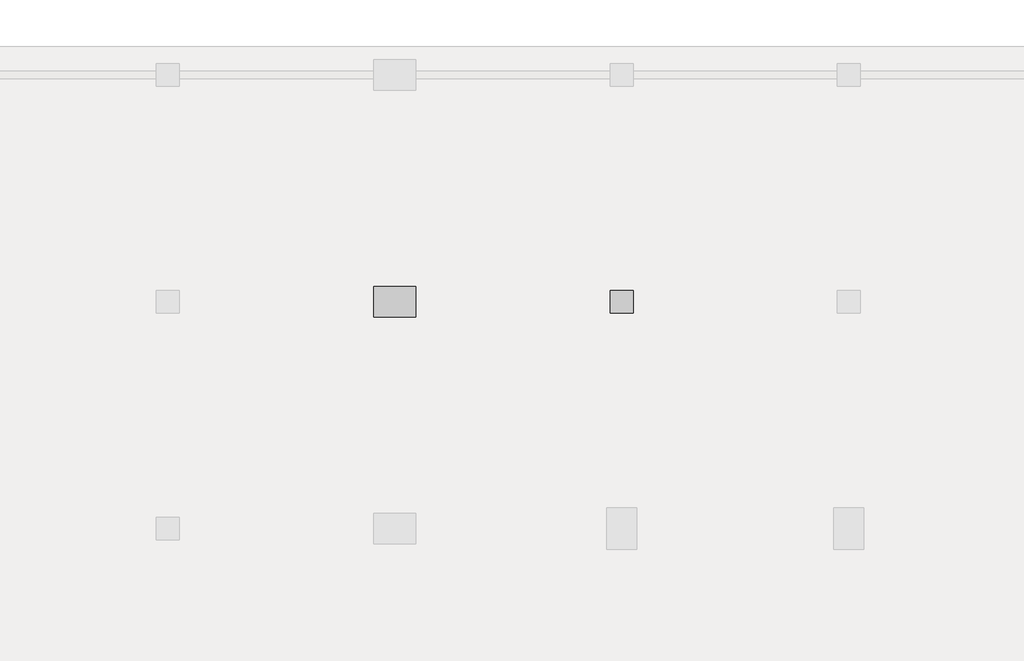
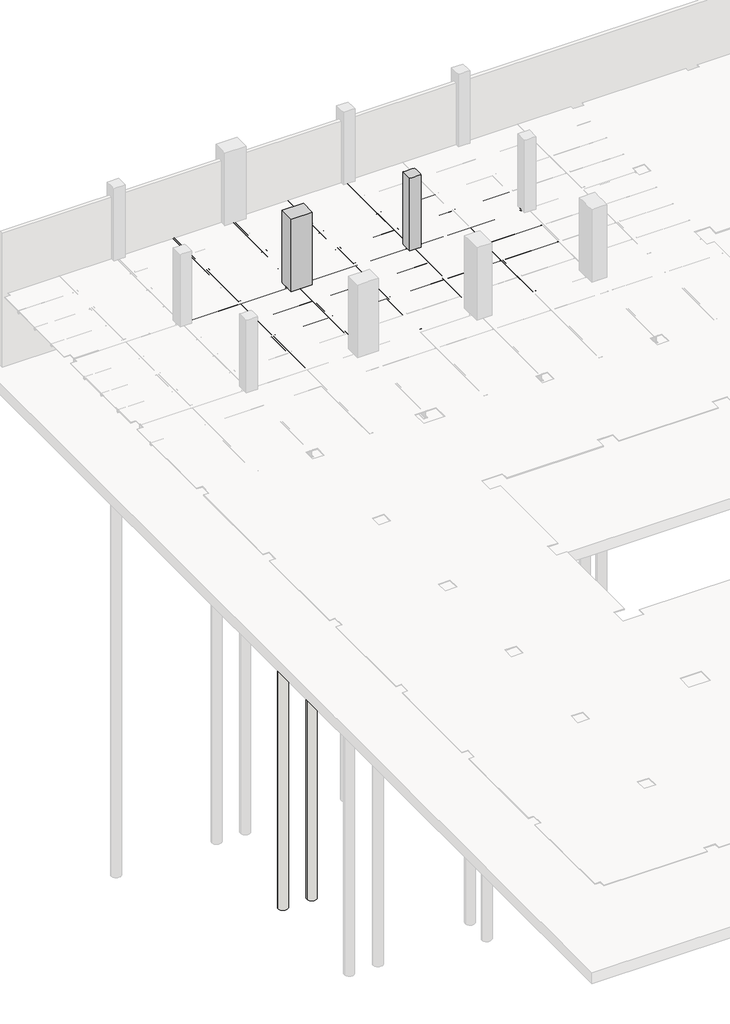
# Not in any storey, part 12 of 16: 31 beams, 2 columns, 2 slabs.
"""IFC4 building model written with IfcOpenShell, lengths in millimetres."""

from ifc_helpers import new_model, si_unit, point, frame, frame_2d, origin, place, context, project, spatial, polyline, circle_curve, trimmed, segment, composite_curve, outline, extrude, faceted_brep, element, save

model = new_model("IFC4")

# Units and contexts
model_context = context("Model", 3, world=origin())
ifc_project = project(units=[si_unit("LENGTHUNIT", "METRE", prefix="MILLI")], contexts=[model_context])

# Site, building
site = spatial("IfcSite", under=ifc_project)
building = spatial("IfcBuilding", under=site)

# Beams
placement = place(None, origin())
element("IfcBeam", 1, ObjectType="Steel Framing_H_KS : H_SB_AR_S02_H-400x200x8x13_BSG1", at=placement, inside=building, context=model_context, shape_type="SweptSolid", body=[
    extrude(outline(composite_curve([segment(polyline([(-11900.0, -4187.0381366), (-11900.0, -4200.0381366), (-12100.0, -4200.0381366), (-12100.0, -4187.0381366), (-12020.0, -4187.0381366)]), True, "CONTINUOUS"), segment(trimmed(circle_curve(frame_2d((-12020.0, -4171.0381366)), 16.0), [point((-12020.0, -4187.0381366))], [point((-12004.0, -4171.0381366))], True, "CARTESIAN"), True, "CONTINUOUS"), segment(polyline([(-12004.0, -4171.0381366), (-12004.0, -3829.0381366)]), True, "CONTINUOUS"), segment(trimmed(circle_curve(frame_2d((-12020.0, -3829.0381366)), 16.0), [point((-12004.0, -3829.0381366))], [point((-12020.0, -3813.0381366))], True, "CARTESIAN"), True, "CONTINUOUS"), segment(polyline([(-12020.0, -3813.0381366), (-12100.0, -3813.0381366), (-12100.0, -3800.0381366), (-11900.0, -3800.0381366), (-11900.0, -3813.0381366), (-11980.0, -3813.0381366)]), True, "CONTINUOUS"), segment(trimmed(circle_curve(frame_2d((-11980.0, -3829.0381366)), 16.0), [point((-11980.0, -3813.0381366))], [point((-11996.0, -3829.0381366))], True, "CARTESIAN"), True, "CONTINUOUS"), segment(polyline([(-11996.0, -3829.0381366), (-11996.0, -4171.0381366)]), True, "CONTINUOUS"), segment(trimmed(circle_curve(frame_2d((-11980.0, -4171.0381366)), 16.0), [point((-11996.0, -4171.0381366))], [point((-11980.0, -4187.0381366))], True, "CARTESIAN"), True, "CONTINUOUS"), segment(polyline([(-11980.0, -4187.0381366), (-11900.0, -4187.0381366)]), True, "CONTINUOUS")], self_intersect=False)), frame((30312.7, 0.0, 0.0), z_axis=(1.0, 0.0, 0.0), x_axis=(0.0, 1.0, 0.0)), (0.0, 0.0, 1.0), 5124.6),
])
element("IfcBeam", 2, ObjectType="Steel Framing_H_KS : H_SB_AR_S02_H-400x200x8x13_BSG2", at=placement, inside=building, context=model_context, shape_type="SweptSolid", body=[
    extrude(outline(composite_curve([segment(polyline([(-4187.0381366, 35900.0), (-4200.0381366, 35900.0), (-4200.0381366, 36100.0), (-4187.0381366, 36100.0), (-4187.0381366, 36020.0)]), True, "CONTINUOUS"), segment(trimmed(circle_curve(frame_2d((-4171.0381366, 36020.0)), 16.0), [point((-4187.0381366, 36020.0))], [point((-4171.0381366, 36004.0))], True, "CARTESIAN"), True, "CONTINUOUS"), segment(polyline([(-4171.0381366, 36004.0), (-3829.0381366, 36004.0)]), True, "CONTINUOUS"), segment(trimmed(circle_curve(frame_2d((-3829.0381366, 36020.0)), 16.0), [point((-3829.0381366, 36004.0))], [point((-3813.0381366, 36020.0))], True, "CARTESIAN"), True, "CONTINUOUS"), segment(polyline([(-3813.0381366, 36020.0), (-3813.0381366, 36100.0), (-3800.0381366, 36100.0), (-3800.0381366, 35900.0), (-3813.0381366, 35900.0), (-3813.0381366, 35980.0)]), True, "CONTINUOUS"), segment(trimmed(circle_curve(frame_2d((-3829.0381366, 35980.0)), 16.0), [point((-3813.0381366, 35980.0))], [point((-3829.0381366, 35996.0))], True, "CARTESIAN"), True, "CONTINUOUS"), segment(polyline([(-3829.0381366, 35996.0), (-4171.0381366, 35996.0)]), True, "CONTINUOUS"), segment(trimmed(circle_curve(frame_2d((-4171.0381366, 35980.0)), 16.0), [point((-4171.0381366, 35996.0))], [point((-4187.0381366, 35980.0))], True, "CARTESIAN"), True, "CONTINUOUS"), segment(polyline([(-4187.0381366, 35980.0), (-4187.0381366, 35900.0)]), True, "CONTINUOUS")], self_intersect=False)), frame((0.0, -11587.3, 0.0), z_axis=(0.0, 1.0, 0.0), x_axis=(0.0, 0.0, 1.0)), (0.0, 0.0, 1.0), 5174.6),
])
element("IfcBeam", 3, ObjectType="Steel Framing_H_KS : H_SB_AR_S02_H-400x200x8x13_BSB1", at=placement, inside=building, context=model_context, shape_type="SweptSolid", body=[
    extrude(outline(composite_curve([segment(polyline([(-4187.0381366, 32900.0), (-4200.0381366, 32900.0), (-4200.0381366, 33100.0), (-4187.0381366, 33100.0), (-4187.0381366, 33020.0)]), True, "CONTINUOUS"), segment(trimmed(circle_curve(frame_2d((-4171.0381366, 33020.0)), 16.0), [point((-4187.0381366, 33020.0))], [point((-4171.0381366, 33004.0))], True, "CARTESIAN"), True, "CONTINUOUS"), segment(polyline([(-4171.0381366, 33004.0), (-3829.0381366, 33004.0)]), True, "CONTINUOUS"), segment(trimmed(circle_curve(frame_2d((-3829.0381366, 33020.0)), 16.0), [point((-3829.0381366, 33004.0))], [point((-3813.0381366, 33020.0))], True, "CARTESIAN"), True, "CONTINUOUS"), segment(polyline([(-3813.0381366, 33020.0), (-3813.0381366, 33100.0), (-3800.0381366, 33100.0), (-3800.0381366, 32900.0), (-3813.0381366, 32900.0), (-3813.0381366, 32980.0)]), True, "CONTINUOUS"), segment(trimmed(circle_curve(frame_2d((-3829.0381366, 32980.0)), 16.0), [point((-3813.0381366, 32980.0))], [point((-3829.0381366, 32996.0))], True, "CARTESIAN"), True, "CONTINUOUS"), segment(polyline([(-3829.0381366, 32996.0), (-4171.0381366, 32996.0)]), True, "CONTINUOUS"), segment(trimmed(circle_curve(frame_2d((-4171.0381366, 32980.0)), 16.0), [point((-4171.0381366, 32996.0))], [point((-4187.0381366, 32980.0))], True, "CARTESIAN"), True, "CONTINUOUS"), segment(polyline([(-4187.0381366, 32980.0), (-4187.0381366, 32900.0)]), True, "CONTINUOUS")], self_intersect=False)), frame((0.0, -11887.3, 0.0), z_axis=(0.0, 1.0, 0.0), x_axis=(0.0, 0.0, 1.0)), (0.0, 0.0, 1.0), 5887.3),
])
element("IfcBeam", 4, ObjectType="Steel Framing_C_KS : H_SB_AR_S02_C-150x75x6.5x10_J1", at=placement, inside=building, context=model_context, shape_type="SweptSolid", body=[
    extrude(outline(composite_curve([segment(polyline([(-8977.2, -3800.0381366), (-8977.2, -3950.0381366), (-9052.2, -3950.0381366)]), True, "CONTINUOUS"), segment(trimmed(circle_curve(frame_2d((-9042.2, -3950.0381366)), 10.0), [point((-9052.2, -3950.0381366))], [point((-9042.2, -3940.0381366))], False, "CARTESIAN"), True, "CONTINUOUS"), segment(polyline([(-9042.2, -3940.0381366), (-8983.7, -3930.7726469), (-8983.7, -3819.3036264), (-9042.2, -3810.0381366)]), True, "CONTINUOUS"), segment(trimmed(circle_curve(frame_2d((-9042.2, -3800.0381366)), 10.0), [point((-9042.2, -3810.0381366))], [point((-9052.2, -3800.0381366))], False, "CARTESIAN"), True, "CONTINUOUS"), segment(polyline([(-9052.2, -3800.0381366), (-8977.2, -3800.0381366)]), True, "CONTINUOUS")], self_intersect=False)), frame((33112.7, 0.0, 0.0), z_axis=(1.0, 0.0, 0.0), x_axis=(0.0, 1.0, 0.0)), (0.0, 0.0, 1.0), 2774.6),
])
element("IfcBeam", 5, ObjectType="Steel Framing_C_KS : H_SB_AR_S02_C-150x75x6.5x10_J1", at=placement, inside=building, context=model_context, shape_type="SweptSolid", body=[
    extrude(outline(composite_curve([segment(polyline([(-10477.2, -3800.0381366), (-10477.2, -3950.0381366), (-10552.2, -3950.0381366)]), True, "CONTINUOUS"), segment(trimmed(circle_curve(frame_2d((-10542.2, -3950.0381366)), 10.0), [point((-10552.2, -3950.0381366))], [point((-10542.2, -3940.0381366))], False, "CARTESIAN"), True, "CONTINUOUS"), segment(polyline([(-10542.2, -3940.0381366), (-10483.7, -3930.7726469), (-10483.7, -3819.3036264), (-10542.2, -3810.0381366)]), True, "CONTINUOUS"), segment(trimmed(circle_curve(frame_2d((-10542.2, -3800.0381366)), 10.0), [point((-10542.2, -3810.0381366))], [point((-10552.2, -3800.0381366))], False, "CARTESIAN"), True, "CONTINUOUS"), segment(polyline([(-10552.2, -3800.0381366), (-10477.2, -3800.0381366)]), True, "CONTINUOUS")], self_intersect=False)), frame((33112.7, 0.0, 0.0), z_axis=(1.0, 0.0, 0.0), x_axis=(0.0, 1.0, 0.0)), (0.0, 0.0, 1.0), 2774.6),
])
element("IfcBeam", 6, ObjectType="Steel Framing_H_KS : H_SB_AR_S02_H-400x200x8x13_BSG1", at=placement, inside=building, context=model_context, shape_type="SweptSolid", body=[
    extrude(outline(composite_curve([segment(polyline([(-11900.0, -4187.0381366), (-11900.0, -4200.0381366), (-12100.0, -4200.0381366), (-12100.0, -4187.0381366), (-12020.0, -4187.0381366)]), True, "CONTINUOUS"), segment(trimmed(circle_curve(frame_2d((-12020.0, -4171.0381366)), 16.0), [point((-12020.0, -4187.0381366))], [point((-12004.0, -4171.0381366))], True, "CARTESIAN"), True, "CONTINUOUS"), segment(polyline([(-12004.0, -4171.0381366), (-12004.0, -3829.0381366)]), True, "CONTINUOUS"), segment(trimmed(circle_curve(frame_2d((-12020.0, -3829.0381366)), 16.0), [point((-12004.0, -3829.0381366))], [point((-12020.0, -3813.0381366))], True, "CARTESIAN"), True, "CONTINUOUS"), segment(polyline([(-12020.0, -3813.0381366), (-12100.0, -3813.0381366), (-12100.0, -3800.0381366), (-11900.0, -3800.0381366), (-11900.0, -3813.0381366), (-11980.0, -3813.0381366)]), True, "CONTINUOUS"), segment(trimmed(circle_curve(frame_2d((-11980.0, -3829.0381366)), 16.0), [point((-11980.0, -3813.0381366))], [point((-11996.0, -3829.0381366))], True, "CARTESIAN"), True, "CONTINUOUS"), segment(polyline([(-11996.0, -3829.0381366), (-11996.0, -4171.0381366)]), True, "CONTINUOUS"), segment(trimmed(circle_curve(frame_2d((-11980.0, -4171.0381366)), 16.0), [point((-11996.0, -4171.0381366))], [point((-11980.0, -4187.0381366))], True, "CARTESIAN"), True, "CONTINUOUS"), segment(polyline([(-11980.0, -4187.0381366), (-11900.0, -4187.0381366)]), True, "CONTINUOUS")], self_intersect=False)), frame((36562.7, 0.0, 0.0), z_axis=(1.0, 0.0, 0.0), x_axis=(0.0, 1.0, 0.0)), (0.0, 0.0, 1.0), 5124.6),
])
element("IfcBeam", 7, ObjectType="Steel Framing_H_KS : H_SB_AR_S02_H-400x200x8x13_BSG2", at=placement, inside=building, context=model_context, shape_type="SweptSolid", body=[
    extrude(outline(composite_curve([segment(polyline([(-4187.0381366, 41900.0), (-4200.0381366, 41900.0), (-4200.0381366, 42100.0), (-4187.0381366, 42100.0), (-4187.0381366, 42020.0)]), True, "CONTINUOUS"), segment(trimmed(circle_curve(frame_2d((-4171.0381366, 42020.0)), 16.0), [point((-4187.0381366, 42020.0))], [point((-4171.0381366, 42004.0))], True, "CARTESIAN"), True, "CONTINUOUS"), segment(polyline([(-4171.0381366, 42004.0), (-3829.0381366, 42004.0)]), True, "CONTINUOUS"), segment(trimmed(circle_curve(frame_2d((-3829.0381366, 42020.0)), 16.0), [point((-3829.0381366, 42004.0))], [point((-3813.0381366, 42020.0))], True, "CARTESIAN"), True, "CONTINUOUS"), segment(polyline([(-3813.0381366, 42020.0), (-3813.0381366, 42100.0), (-3800.0381366, 42100.0), (-3800.0381366, 41900.0), (-3813.0381366, 41900.0), (-3813.0381366, 41980.0)]), True, "CONTINUOUS"), segment(trimmed(circle_curve(frame_2d((-3829.0381366, 41980.0)), 16.0), [point((-3813.0381366, 41980.0))], [point((-3829.0381366, 41996.0))], True, "CARTESIAN"), True, "CONTINUOUS"), segment(polyline([(-3829.0381366, 41996.0), (-4171.0381366, 41996.0)]), True, "CONTINUOUS"), segment(trimmed(circle_curve(frame_2d((-4171.0381366, 41980.0)), 16.0), [point((-4171.0381366, 41996.0))], [point((-4187.0381366, 41980.0))], True, "CARTESIAN"), True, "CONTINUOUS"), segment(polyline([(-4187.0381366, 41980.0), (-4187.0381366, 41900.0)]), True, "CONTINUOUS")], self_intersect=False)), frame((0.0, -11687.3, 0.0), z_axis=(0.0, 1.0, 0.0), x_axis=(0.0, 0.0, 1.0)), (0.0, 0.0, 1.0), 5374.6),
])
element("IfcBeam", 8, ObjectType="Steel Framing_H_KS : H_SB_AR_S02_H-400x200x8x13_BSB1", at=placement, inside=building, context=model_context, shape_type="SweptSolid", body=[
    extrude(outline(composite_curve([segment(polyline([(-4187.0381366, 38900.0), (-4200.0381366, 38900.0), (-4200.0381366, 39100.0), (-4187.0381366, 39100.0), (-4187.0381366, 39020.0)]), True, "CONTINUOUS"), segment(trimmed(circle_curve(frame_2d((-4171.0381366, 39020.0)), 16.0), [point((-4187.0381366, 39020.0))], [point((-4171.0381366, 39004.0))], True, "CARTESIAN"), True, "CONTINUOUS"), segment(polyline([(-4171.0381366, 39004.0), (-3829.0381366, 39004.0)]), True, "CONTINUOUS"), segment(trimmed(circle_curve(frame_2d((-3829.0381366, 39020.0)), 16.0), [point((-3829.0381366, 39004.0))], [point((-3813.0381366, 39020.0))], True, "CARTESIAN"), True, "CONTINUOUS"), segment(polyline([(-3813.0381366, 39020.0), (-3813.0381366, 39100.0), (-3800.0381366, 39100.0), (-3800.0381366, 38900.0), (-3813.0381366, 38900.0), (-3813.0381366, 38980.0)]), True, "CONTINUOUS"), segment(trimmed(circle_curve(frame_2d((-3829.0381366, 38980.0)), 16.0), [point((-3813.0381366, 38980.0))], [point((-3829.0381366, 38996.0))], True, "CARTESIAN"), True, "CONTINUOUS"), segment(polyline([(-3829.0381366, 38996.0), (-4171.0381366, 38996.0)]), True, "CONTINUOUS"), segment(trimmed(circle_curve(frame_2d((-4171.0381366, 38980.0)), 16.0), [point((-4171.0381366, 38996.0))], [point((-4187.0381366, 38980.0))], True, "CARTESIAN"), True, "CONTINUOUS"), segment(polyline([(-4187.0381366, 38980.0), (-4187.0381366, 38900.0)]), True, "CONTINUOUS")], self_intersect=False)), frame((0.0, -11887.3, 0.0), z_axis=(0.0, 1.0, 0.0), x_axis=(0.0, 0.0, 1.0)), (0.0, 0.0, 1.0), 5887.3),
])
element("IfcBeam", 9, ObjectType="Steel Framing_C_KS : H_SB_AR_S02_C-150x75x6.5x10_J1", at=placement, inside=building, context=model_context, shape_type="SweptSolid", body=[
    extrude(outline(composite_curve([segment(polyline([(-8977.2, -3800.0381366), (-8977.2, -3950.0381366), (-9052.2, -3950.0381366)]), True, "CONTINUOUS"), segment(trimmed(circle_curve(frame_2d((-9042.2, -3950.0381366)), 10.0), [point((-9052.2, -3950.0381366))], [point((-9042.2, -3940.0381366))], False, "CARTESIAN"), True, "CONTINUOUS"), segment(polyline([(-9042.2, -3940.0381366), (-8983.7, -3930.7726469), (-8983.7, -3819.3036264), (-9042.2, -3810.0381366)]), True, "CONTINUOUS"), segment(trimmed(circle_curve(frame_2d((-9042.2, -3800.0381366)), 10.0), [point((-9042.2, -3810.0381366))], [point((-9052.2, -3800.0381366))], False, "CARTESIAN"), True, "CONTINUOUS"), segment(polyline([(-9052.2, -3800.0381366), (-8977.2, -3800.0381366)]), True, "CONTINUOUS")], self_intersect=False)), frame((36112.7, 0.0, 0.0), z_axis=(1.0, 0.0, 0.0), x_axis=(0.0, 1.0, 0.0)), (0.0, 0.0, 1.0), 2774.6),
])
element("IfcBeam", 10, ObjectType="Steel Framing_C_KS : H_SB_AR_S02_C-150x75x6.5x10_J1", at=placement, inside=building, context=model_context, shape_type="SweptSolid", body=[
    extrude(outline(composite_curve([segment(polyline([(-10477.2, -3800.0381366), (-10477.2, -3950.0381366), (-10552.2, -3950.0381366)]), True, "CONTINUOUS"), segment(trimmed(circle_curve(frame_2d((-10542.2, -3950.0381366)), 10.0), [point((-10552.2, -3950.0381366))], [point((-10542.2, -3940.0381366))], False, "CARTESIAN"), True, "CONTINUOUS"), segment(polyline([(-10542.2, -3940.0381366), (-10483.7, -3930.7726469), (-10483.7, -3819.3036264), (-10542.2, -3810.0381366)]), True, "CONTINUOUS"), segment(trimmed(circle_curve(frame_2d((-10542.2, -3800.0381366)), 10.0), [point((-10542.2, -3810.0381366))], [point((-10552.2, -3800.0381366))], False, "CARTESIAN"), True, "CONTINUOUS"), segment(polyline([(-10552.2, -3800.0381366), (-10477.2, -3800.0381366)]), True, "CONTINUOUS")], self_intersect=False)), frame((36112.7, 0.0, 0.0), z_axis=(1.0, 0.0, 0.0), x_axis=(0.0, 1.0, 0.0)), (0.0, 0.0, 1.0), 2774.6),
])
element("IfcBeam", 11, ObjectType="Steel Framing_C_KS : H_SB_AR_S02_C-150x75x6.5x10_J1", at=placement, inside=building, context=model_context, shape_type="SweptSolid", body=[
    extrude(outline(composite_curve([segment(polyline([(-8977.2, -3800.0381366), (-8977.2, -3950.0381366), (-9052.2, -3950.0381366)]), True, "CONTINUOUS"), segment(trimmed(circle_curve(frame_2d((-9042.2, -3950.0381366)), 10.0), [point((-9052.2, -3950.0381366))], [point((-9042.2, -3940.0381366))], False, "CARTESIAN"), True, "CONTINUOUS"), segment(polyline([(-9042.2, -3940.0381366), (-8983.7, -3930.7726469), (-8983.7, -3819.3036264), (-9042.2, -3810.0381366)]), True, "CONTINUOUS"), segment(trimmed(circle_curve(frame_2d((-9042.2, -3800.0381366)), 10.0), [point((-9042.2, -3810.0381366))], [point((-9052.2, -3800.0381366))], False, "CARTESIAN"), True, "CONTINUOUS"), segment(polyline([(-9052.2, -3800.0381366), (-8977.2, -3800.0381366)]), True, "CONTINUOUS")], self_intersect=False)), frame((39112.7, 0.0, 0.0), z_axis=(1.0, 0.0, 0.0), x_axis=(0.0, 1.0, 0.0)), (0.0, 0.0, 1.0), 2774.6),
])
element("IfcBeam", 12, ObjectType="Steel Framing_C_KS : H_SB_AR_S02_C-150x75x6.5x10_J1", at=placement, inside=building, context=model_context, shape_type="SweptSolid", body=[
    extrude(outline(composite_curve([segment(polyline([(-10477.2, -3800.0381366), (-10477.2, -3950.0381366), (-10552.2, -3950.0381366)]), True, "CONTINUOUS"), segment(trimmed(circle_curve(frame_2d((-10542.2, -3950.0381366)), 10.0), [point((-10552.2, -3950.0381366))], [point((-10542.2, -3940.0381366))], False, "CARTESIAN"), True, "CONTINUOUS"), segment(polyline([(-10542.2, -3940.0381366), (-10483.7, -3930.7726469), (-10483.7, -3819.3036264), (-10542.2, -3810.0381366)]), True, "CONTINUOUS"), segment(trimmed(circle_curve(frame_2d((-10542.2, -3800.0381366)), 10.0), [point((-10542.2, -3810.0381366))], [point((-10552.2, -3800.0381366))], False, "CARTESIAN"), True, "CONTINUOUS"), segment(polyline([(-10552.2, -3800.0381366), (-10477.2, -3800.0381366)]), True, "CONTINUOUS")], self_intersect=False)), frame((39112.7, 0.0, 0.0), z_axis=(1.0, 0.0, 0.0), x_axis=(0.0, 1.0, 0.0)), (0.0, 0.0, 1.0), 2774.6),
])
element("IfcBeam", 13, ObjectType="Steel Framing_H_KS : H_SB_AR_S02_H-400x200x8x13_BSG1", at=placement, inside=building, context=model_context, shape_type="SweptSolid", body=[
    extrude(outline(composite_curve([segment(polyline([(-11900.0, -4187.0381366), (-11900.0, -4200.0381366), (-12100.0, -4200.0381366), (-12100.0, -4187.0381366), (-12020.0, -4187.0381366)]), True, "CONTINUOUS"), segment(trimmed(circle_curve(frame_2d((-12020.0, -4171.0381366)), 16.0), [point((-12020.0, -4187.0381366))], [point((-12004.0, -4171.0381366))], True, "CARTESIAN"), True, "CONTINUOUS"), segment(polyline([(-12004.0, -4171.0381366), (-12004.0, -3829.0381366)]), True, "CONTINUOUS"), segment(trimmed(circle_curve(frame_2d((-12020.0, -3829.0381366)), 16.0), [point((-12004.0, -3829.0381366))], [point((-12020.0, -3813.0381366))], True, "CARTESIAN"), True, "CONTINUOUS"), segment(polyline([(-12020.0, -3813.0381366), (-12100.0, -3813.0381366), (-12100.0, -3800.0381366), (-11900.0, -3800.0381366), (-11900.0, -3813.0381366), (-11980.0, -3813.0381366)]), True, "CONTINUOUS"), segment(trimmed(circle_curve(frame_2d((-11980.0, -3829.0381366)), 16.0), [point((-11980.0, -3813.0381366))], [point((-11996.0, -3829.0381366))], True, "CARTESIAN"), True, "CONTINUOUS"), segment(polyline([(-11996.0, -3829.0381366), (-11996.0, -4171.0381366)]), True, "CONTINUOUS"), segment(trimmed(circle_curve(frame_2d((-11980.0, -4171.0381366)), 16.0), [point((-11996.0, -4171.0381366))], [point((-11980.0, -4187.0381366))], True, "CARTESIAN"), True, "CONTINUOUS"), segment(polyline([(-11980.0, -4187.0381366), (-11900.0, -4187.0381366)]), True, "CONTINUOUS")], self_intersect=False)), frame((42312.7, 0.0, 0.0), z_axis=(1.0, 0.0, 0.0), x_axis=(0.0, 1.0, 0.0)), (0.0, 0.0, 1.0), 5374.6),
])
element("IfcBeam", 14, ObjectType="Steel Framing_C_KS : H_SB_AR_S02_C-150x75x6.5x10_J1", at=placement, inside=building, context=model_context, shape_type="SweptSolid", body=[
    extrude(outline(composite_curve([segment(polyline([(-8977.2, -3800.0381366), (-8977.2, -3950.0381366), (-9052.2, -3950.0381366)]), True, "CONTINUOUS"), segment(trimmed(circle_curve(frame_2d((-9042.2, -3950.0381366)), 10.0), [point((-9052.2, -3950.0381366))], [point((-9042.2, -3940.0381366))], False, "CARTESIAN"), True, "CONTINUOUS"), segment(polyline([(-9042.2, -3940.0381366), (-8983.7, -3930.7726469), (-8983.7, -3819.3036264), (-9042.2, -3810.0381366)]), True, "CONTINUOUS"), segment(trimmed(circle_curve(frame_2d((-9042.2, -3800.0381366)), 10.0), [point((-9042.2, -3810.0381366))], [point((-9052.2, -3800.0381366))], False, "CARTESIAN"), True, "CONTINUOUS"), segment(polyline([(-9052.2, -3800.0381366), (-8977.2, -3800.0381366)]), True, "CONTINUOUS")], self_intersect=False)), frame((42112.7, 0.0, 0.0), z_axis=(1.0, 0.0, 0.0), x_axis=(0.0, 1.0, 0.0)), (0.0, 0.0, 1.0), 2774.6),
])
element("IfcBeam", 15, ObjectType="Steel Framing_C_KS : H_SB_AR_S02_C-150x75x6.5x10_J1", at=placement, inside=building, context=model_context, shape_type="SweptSolid", body=[
    extrude(outline(composite_curve([segment(polyline([(-10477.2, -3800.0381366), (-10477.2, -3950.0381366), (-10552.2, -3950.0381366)]), True, "CONTINUOUS"), segment(trimmed(circle_curve(frame_2d((-10542.2, -3950.0381366)), 10.0), [point((-10552.2, -3950.0381366))], [point((-10542.2, -3940.0381366))], False, "CARTESIAN"), True, "CONTINUOUS"), segment(polyline([(-10542.2, -3940.0381366), (-10483.7, -3930.7726469), (-10483.7, -3819.3036264), (-10542.2, -3810.0381366)]), True, "CONTINUOUS"), segment(trimmed(circle_curve(frame_2d((-10542.2, -3800.0381366)), 10.0), [point((-10542.2, -3810.0381366))], [point((-10552.2, -3800.0381366))], False, "CARTESIAN"), True, "CONTINUOUS"), segment(polyline([(-10552.2, -3800.0381366), (-10477.2, -3800.0381366)]), True, "CONTINUOUS")], self_intersect=False)), frame((42112.7, 0.0, 0.0), z_axis=(1.0, 0.0, 0.0), x_axis=(0.0, 1.0, 0.0)), (0.0, 0.0, 1.0), 2774.6),
])
element("IfcBeam", 16, ObjectType="Steel Framing_C_KS : H_SB_AR_S02_C-150x75x6.5x10_J1", at=placement, inside=building, context=model_context, shape_type="SweptSolid", body=[
    extrude(outline(composite_curve([segment(polyline([(-10477.2, -3800.0381366), (-10477.2, -3950.0381366), (-10552.2, -3950.0381366)]), True, "CONTINUOUS"), segment(trimmed(circle_curve(frame_2d((-10542.2, -3950.0381366)), 10.0), [point((-10552.2, -3950.0381366))], [point((-10542.2, -3940.0381366))], False, "CARTESIAN"), True, "CONTINUOUS"), segment(polyline([(-10542.2, -3940.0381366), (-10483.7, -3930.7726469), (-10483.7, -3819.3036264), (-10542.2, -3810.0381366)]), True, "CONTINUOUS"), segment(trimmed(circle_curve(frame_2d((-10542.2, -3800.0381366)), 10.0), [point((-10542.2, -3810.0381366))], [point((-10552.2, -3800.0381366))], False, "CARTESIAN"), True, "CONTINUOUS"), segment(polyline([(-10552.2, -3800.0381366), (-10477.2, -3800.0381366)]), True, "CONTINUOUS")], self_intersect=False)), frame((45112.7, 0.0, 0.0), z_axis=(1.0, 0.0, 0.0), x_axis=(0.0, 1.0, 0.0)), (0.0, 0.0, 1.0), 2774.6),
])
element("IfcBeam", 17, ObjectType="Steel Framing_H_KS : H_SB_AR_S02_H-400x200x8x13_BSG2", at=placement, inside=building, context=model_context, shape_type="SweptSolid", body=[
    extrude(outline(composite_curve([segment(polyline([(-4187.0381366, 35900.0), (-4200.0381366, 35900.0), (-4200.0381366, 36100.0), (-4187.0381366, 36100.0), (-4187.0381366, 36020.0)]), True, "CONTINUOUS"), segment(trimmed(circle_curve(frame_2d((-4171.0381366, 36020.0)), 16.0), [point((-4187.0381366, 36020.0))], [point((-4171.0381366, 36004.0))], True, "CARTESIAN"), True, "CONTINUOUS"), segment(polyline([(-4171.0381366, 36004.0), (-3829.0381366, 36004.0)]), True, "CONTINUOUS"), segment(trimmed(circle_curve(frame_2d((-3829.0381366, 36020.0)), 16.0), [point((-3829.0381366, 36004.0))], [point((-3813.0381366, 36020.0))], True, "CARTESIAN"), True, "CONTINUOUS"), segment(polyline([(-3813.0381366, 36020.0), (-3813.0381366, 36100.0), (-3800.0381366, 36100.0), (-3800.0381366, 35900.0), (-3813.0381366, 35900.0), (-3813.0381366, 35980.0)]), True, "CONTINUOUS"), segment(trimmed(circle_curve(frame_2d((-3829.0381366, 35980.0)), 16.0), [point((-3813.0381366, 35980.0))], [point((-3829.0381366, 35996.0))], True, "CARTESIAN"), True, "CONTINUOUS"), segment(polyline([(-3829.0381366, 35996.0), (-4171.0381366, 35996.0)]), True, "CONTINUOUS"), segment(trimmed(circle_curve(frame_2d((-4171.0381366, 35980.0)), 16.0), [point((-4171.0381366, 35996.0))], [point((-4187.0381366, 35980.0))], True, "CARTESIAN"), True, "CONTINUOUS"), segment(polyline([(-4187.0381366, 35980.0), (-4187.0381366, 35900.0)]), True, "CONTINUOUS")], self_intersect=False)), frame((0.0, -17587.3, 0.0), z_axis=(0.0, 1.0, 0.0), x_axis=(0.0, 0.0, 1.0)), (0.0, 0.0, 1.0), 5174.6),
])
element("IfcBeam", 18, ObjectType="Steel Framing_H_KS : H_SB_AR_S02_H-400x200x8x13_BSB1", at=placement, inside=building, context=model_context, shape_type="SweptSolid", body=[
    extrude(outline(composite_curve([segment(polyline([(-4187.0381366, 32900.0), (-4200.0381366, 32900.0), (-4200.0381366, 33100.0), (-4187.0381366, 33100.0), (-4187.0381366, 33020.0)]), True, "CONTINUOUS"), segment(trimmed(circle_curve(frame_2d((-4171.0381366, 33020.0)), 16.0), [point((-4187.0381366, 33020.0))], [point((-4171.0381366, 33004.0))], True, "CARTESIAN"), True, "CONTINUOUS"), segment(polyline([(-4171.0381366, 33004.0), (-3829.0381366, 33004.0)]), True, "CONTINUOUS"), segment(trimmed(circle_curve(frame_2d((-3829.0381366, 33020.0)), 16.0), [point((-3829.0381366, 33004.0))], [point((-3813.0381366, 33020.0))], True, "CARTESIAN"), True, "CONTINUOUS"), segment(polyline([(-3813.0381366, 33020.0), (-3813.0381366, 33100.0), (-3800.0381366, 33100.0), (-3800.0381366, 32900.0), (-3813.0381366, 32900.0), (-3813.0381366, 32980.0)]), True, "CONTINUOUS"), segment(trimmed(circle_curve(frame_2d((-3829.0381366, 32980.0)), 16.0), [point((-3813.0381366, 32980.0))], [point((-3829.0381366, 32996.0))], True, "CARTESIAN"), True, "CONTINUOUS"), segment(polyline([(-3829.0381366, 32996.0), (-4171.0381366, 32996.0)]), True, "CONTINUOUS"), segment(trimmed(circle_curve(frame_2d((-4171.0381366, 32980.0)), 16.0), [point((-4171.0381366, 32996.0))], [point((-4187.0381366, 32980.0))], True, "CARTESIAN"), True, "CONTINUOUS"), segment(polyline([(-4187.0381366, 32980.0), (-4187.0381366, 32900.0)]), True, "CONTINUOUS")], self_intersect=False)), frame((0.0, -17887.3, 0.0), z_axis=(0.0, 1.0, 0.0), x_axis=(0.0, 0.0, 1.0)), (0.0, 0.0, 1.0), 5774.6),
])
element("IfcBeam", 19, ObjectType="Steel Framing_C_KS : H_SB_AR_S02_C-150x75x6.5x10_J1", at=placement, inside=building, context=model_context, shape_type="SweptSolid", body=[
    extrude(outline(composite_curve([segment(polyline([(-14977.2, -3800.0381366), (-14977.2, -3950.0381366), (-15052.2, -3950.0381366)]), True, "CONTINUOUS"), segment(trimmed(circle_curve(frame_2d((-15042.2, -3950.0381366)), 10.0), [point((-15052.2, -3950.0381366))], [point((-15042.2, -3940.0381366))], False, "CARTESIAN"), True, "CONTINUOUS"), segment(polyline([(-15042.2, -3940.0381366), (-14983.7, -3930.7726469), (-14983.7, -3819.3036264), (-15042.2, -3810.0381366)]), True, "CONTINUOUS"), segment(trimmed(circle_curve(frame_2d((-15042.2, -3800.0381366)), 10.0), [point((-15042.2, -3810.0381366))], [point((-15052.2, -3800.0381366))], False, "CARTESIAN"), True, "CONTINUOUS"), segment(polyline([(-15052.2, -3800.0381366), (-14977.2, -3800.0381366)]), True, "CONTINUOUS")], self_intersect=False)), frame((33112.7, 0.0, 0.0), z_axis=(1.0, 0.0, 0.0), x_axis=(0.0, 1.0, 0.0)), (0.0, 0.0, 1.0), 2774.6),
])
element("IfcBeam", 20, ObjectType="Steel Framing_C_KS : H_SB_AR_S02_C-150x75x6.5x10_J1", at=placement, inside=building, context=model_context, shape_type="SweptSolid", body=[
    extrude(outline(composite_curve([segment(polyline([(-13477.2, -3800.0381366), (-13477.2, -3950.0381366), (-13552.2, -3950.0381366)]), True, "CONTINUOUS"), segment(trimmed(circle_curve(frame_2d((-13542.2, -3950.0381366)), 10.0), [point((-13552.2, -3950.0381366))], [point((-13542.2, -3940.0381366))], False, "CARTESIAN"), True, "CONTINUOUS"), segment(polyline([(-13542.2, -3940.0381366), (-13483.7, -3930.7726469), (-13483.7, -3819.3036264), (-13542.2, -3810.0381366)]), True, "CONTINUOUS"), segment(trimmed(circle_curve(frame_2d((-13542.2, -3800.0381366)), 10.0), [point((-13542.2, -3810.0381366))], [point((-13552.2, -3800.0381366))], False, "CARTESIAN"), True, "CONTINUOUS"), segment(polyline([(-13552.2, -3800.0381366), (-13477.2, -3800.0381366)]), True, "CONTINUOUS")], self_intersect=False)), frame((33112.7, 0.0, 0.0), z_axis=(1.0, 0.0, 0.0), x_axis=(0.0, 1.0, 0.0)), (0.0, 0.0, 1.0), 2774.6),
])
element("IfcBeam", 21, ObjectType="Steel Framing_H_KS : H_SB_AR_S02_H-400x200x8x13_BSG2", at=placement, inside=building, context=model_context, shape_type="SweptSolid", body=[
    extrude(outline(composite_curve([segment(polyline([(-4187.0381366, 41900.0), (-4200.0381366, 41900.0), (-4200.0381366, 42100.0), (-4187.0381366, 42100.0), (-4187.0381366, 42020.0)]), True, "CONTINUOUS"), segment(trimmed(circle_curve(frame_2d((-4171.0381366, 42020.0)), 16.0), [point((-4187.0381366, 42020.0))], [point((-4171.0381366, 42004.0))], True, "CARTESIAN"), True, "CONTINUOUS"), segment(polyline([(-4171.0381366, 42004.0), (-3829.0381366, 42004.0)]), True, "CONTINUOUS"), segment(trimmed(circle_curve(frame_2d((-3829.0381366, 42020.0)), 16.0), [point((-3829.0381366, 42004.0))], [point((-3813.0381366, 42020.0))], True, "CARTESIAN"), True, "CONTINUOUS"), segment(polyline([(-3813.0381366, 42020.0), (-3813.0381366, 42100.0), (-3800.0381366, 42100.0), (-3800.0381366, 41900.0), (-3813.0381366, 41900.0), (-3813.0381366, 41980.0)]), True, "CONTINUOUS"), segment(trimmed(circle_curve(frame_2d((-3829.0381366, 41980.0)), 16.0), [point((-3813.0381366, 41980.0))], [point((-3829.0381366, 41996.0))], True, "CARTESIAN"), True, "CONTINUOUS"), segment(polyline([(-3829.0381366, 41996.0), (-4171.0381366, 41996.0)]), True, "CONTINUOUS"), segment(trimmed(circle_curve(frame_2d((-4171.0381366, 41980.0)), 16.0), [point((-4171.0381366, 41996.0))], [point((-4187.0381366, 41980.0))], True, "CARTESIAN"), True, "CONTINUOUS"), segment(polyline([(-4187.0381366, 41980.0), (-4187.0381366, 41900.0)]), True, "CONTINUOUS")], self_intersect=False)), frame((0.0, -17437.3, 0.0), z_axis=(0.0, 1.0, 0.0), x_axis=(0.0, 0.0, 1.0)), (0.0, 0.0, 1.0), 5124.6),
])
element("IfcBeam", 22, ObjectType="Steel Framing_H_KS : H_SB_AR_S02_H-400x200x8x13_BSB1", at=placement, inside=building, context=model_context, shape_type="SweptSolid", body=[
    extrude(outline(composite_curve([segment(polyline([(-4187.0381366, 38900.0), (-4200.0381366, 38900.0), (-4200.0381366, 39100.0), (-4187.0381366, 39100.0), (-4187.0381366, 39020.0)]), True, "CONTINUOUS"), segment(trimmed(circle_curve(frame_2d((-4171.0381366, 39020.0)), 16.0), [point((-4187.0381366, 39020.0))], [point((-4171.0381366, 39004.0))], True, "CARTESIAN"), True, "CONTINUOUS"), segment(polyline([(-4171.0381366, 39004.0), (-3829.0381366, 39004.0)]), True, "CONTINUOUS"), segment(trimmed(circle_curve(frame_2d((-3829.0381366, 39020.0)), 16.0), [point((-3829.0381366, 39004.0))], [point((-3813.0381366, 39020.0))], True, "CARTESIAN"), True, "CONTINUOUS"), segment(polyline([(-3813.0381366, 39020.0), (-3813.0381366, 39100.0), (-3800.0381366, 39100.0), (-3800.0381366, 38900.0), (-3813.0381366, 38900.0), (-3813.0381366, 38980.0)]), True, "CONTINUOUS"), segment(trimmed(circle_curve(frame_2d((-3829.0381366, 38980.0)), 16.0), [point((-3813.0381366, 38980.0))], [point((-3829.0381366, 38996.0))], True, "CARTESIAN"), True, "CONTINUOUS"), segment(polyline([(-3829.0381366, 38996.0), (-4171.0381366, 38996.0)]), True, "CONTINUOUS"), segment(trimmed(circle_curve(frame_2d((-4171.0381366, 38980.0)), 16.0), [point((-4171.0381366, 38996.0))], [point((-4187.0381366, 38980.0))], True, "CARTESIAN"), True, "CONTINUOUS"), segment(polyline([(-4187.0381366, 38980.0), (-4187.0381366, 38900.0)]), True, "CONTINUOUS")], self_intersect=False)), frame((0.0, -17887.3, 0.0), z_axis=(0.0, 1.0, 0.0), x_axis=(0.0, 0.0, 1.0)), (0.0, 0.0, 1.0), 5774.6),
])
element("IfcBeam", 23, ObjectType="Steel Framing_C_KS : H_SB_AR_S02_C-150x75x6.5x10_J1", at=placement, inside=building, context=model_context, shape_type="SweptSolid", body=[
    extrude(outline(composite_curve([segment(polyline([(-14977.2, -3800.0381366), (-14977.2, -3950.0381366), (-15052.2, -3950.0381366)]), True, "CONTINUOUS"), segment(trimmed(circle_curve(frame_2d((-15042.2, -3950.0381366)), 10.0), [point((-15052.2, -3950.0381366))], [point((-15042.2, -3940.0381366))], False, "CARTESIAN"), True, "CONTINUOUS"), segment(polyline([(-15042.2, -3940.0381366), (-14983.7, -3930.7726469), (-14983.7, -3819.3036264), (-15042.2, -3810.0381366)]), True, "CONTINUOUS"), segment(trimmed(circle_curve(frame_2d((-15042.2, -3800.0381366)), 10.0), [point((-15042.2, -3810.0381366))], [point((-15052.2, -3800.0381366))], False, "CARTESIAN"), True, "CONTINUOUS"), segment(polyline([(-15052.2, -3800.0381366), (-14977.2, -3800.0381366)]), True, "CONTINUOUS")], self_intersect=False)), frame((36112.7, 0.0, 0.0), z_axis=(1.0, 0.0, 0.0), x_axis=(0.0, 1.0, 0.0)), (0.0, 0.0, 1.0), 2774.6),
])
element("IfcBeam", 24, ObjectType="Steel Framing_C_KS : H_SB_AR_S02_C-150x75x6.5x10_J1", at=placement, inside=building, context=model_context, shape_type="SweptSolid", body=[
    extrude(outline(composite_curve([segment(polyline([(-13477.2, -3800.0381366), (-13477.2, -3950.0381366), (-13552.2, -3950.0381366)]), True, "CONTINUOUS"), segment(trimmed(circle_curve(frame_2d((-13542.2, -3950.0381366)), 10.0), [point((-13552.2, -3950.0381366))], [point((-13542.2, -3940.0381366))], False, "CARTESIAN"), True, "CONTINUOUS"), segment(polyline([(-13542.2, -3940.0381366), (-13483.7, -3930.7726469), (-13483.7, -3819.3036264), (-13542.2, -3810.0381366)]), True, "CONTINUOUS"), segment(trimmed(circle_curve(frame_2d((-13542.2, -3800.0381366)), 10.0), [point((-13542.2, -3810.0381366))], [point((-13552.2, -3800.0381366))], False, "CARTESIAN"), True, "CONTINUOUS"), segment(polyline([(-13552.2, -3800.0381366), (-13477.2, -3800.0381366)]), True, "CONTINUOUS")], self_intersect=False)), frame((36112.7, 0.0, 0.0), z_axis=(1.0, 0.0, 0.0), x_axis=(0.0, 1.0, 0.0)), (0.0, 0.0, 1.0), 2774.6),
])
element("IfcBeam", 25, ObjectType="Steel Framing_C_KS : H_SB_AR_S02_C-150x75x6.5x10_J1", at=placement, inside=building, context=model_context, shape_type="SweptSolid", body=[
    extrude(outline(composite_curve([segment(polyline([(-14977.2, -3800.0381366), (-14977.2, -3950.0381366), (-15052.2, -3950.0381366)]), True, "CONTINUOUS"), segment(trimmed(circle_curve(frame_2d((-15042.2, -3950.0381366)), 10.0), [point((-15052.2, -3950.0381366))], [point((-15042.2, -3940.0381366))], False, "CARTESIAN"), True, "CONTINUOUS"), segment(polyline([(-15042.2, -3940.0381366), (-14983.7, -3930.7726469), (-14983.7, -3819.3036264), (-15042.2, -3810.0381366)]), True, "CONTINUOUS"), segment(trimmed(circle_curve(frame_2d((-15042.2, -3800.0381366)), 10.0), [point((-15042.2, -3810.0381366))], [point((-15052.2, -3800.0381366))], False, "CARTESIAN"), True, "CONTINUOUS"), segment(polyline([(-15052.2, -3800.0381366), (-14977.2, -3800.0381366)]), True, "CONTINUOUS")], self_intersect=False)), frame((39112.7, 0.0, 0.0), z_axis=(1.0, 0.0, 0.0), x_axis=(0.0, 1.0, 0.0)), (0.0, 0.0, 1.0), 2774.6),
])
element("IfcBeam", 26, ObjectType="Steel Framing_C_KS : H_SB_AR_S02_C-150x75x6.5x10_J1", at=placement, inside=building, context=model_context, shape_type="SweptSolid", body=[
    extrude(outline(composite_curve([segment(polyline([(-13477.2, -3800.0381366), (-13477.2, -3950.0381366), (-13552.2, -3950.0381366)]), True, "CONTINUOUS"), segment(trimmed(circle_curve(frame_2d((-13542.2, -3950.0381366)), 10.0), [point((-13552.2, -3950.0381366))], [point((-13542.2, -3940.0381366))], False, "CARTESIAN"), True, "CONTINUOUS"), segment(polyline([(-13542.2, -3940.0381366), (-13483.7, -3930.7726469), (-13483.7, -3819.3036264), (-13542.2, -3810.0381366)]), True, "CONTINUOUS"), segment(trimmed(circle_curve(frame_2d((-13542.2, -3800.0381366)), 10.0), [point((-13542.2, -3810.0381366))], [point((-13552.2, -3800.0381366))], False, "CARTESIAN"), True, "CONTINUOUS"), segment(polyline([(-13552.2, -3800.0381366), (-13477.2, -3800.0381366)]), True, "CONTINUOUS")], self_intersect=False)), frame((39112.7, 0.0, 0.0), z_axis=(1.0, 0.0, 0.0), x_axis=(0.0, 1.0, 0.0)), (0.0, 0.0, 1.0), 2774.6),
])
element("IfcBeam", 27, ObjectType="Steel Framing_H_KS : H_SB_AR_S02_H-400x200x8x13_BSB1", at=placement, inside=building, context=model_context, shape_type="SweptSolid", body=[
    extrude(outline(composite_curve([segment(polyline([(-4187.0381366, 44900.0), (-4200.0381366, 44900.0), (-4200.0381366, 45100.0), (-4187.0381366, 45100.0), (-4187.0381366, 45020.0)]), True, "CONTINUOUS"), segment(trimmed(circle_curve(frame_2d((-4171.0381366, 45020.0)), 16.0), [point((-4187.0381366, 45020.0))], [point((-4171.0381366, 45004.0))], True, "CARTESIAN"), True, "CONTINUOUS"), segment(polyline([(-4171.0381366, 45004.0), (-3829.0381366, 45004.0)]), True, "CONTINUOUS"), segment(trimmed(circle_curve(frame_2d((-3829.0381366, 45020.0)), 16.0), [point((-3829.0381366, 45004.0))], [point((-3813.0381366, 45020.0))], True, "CARTESIAN"), True, "CONTINUOUS"), segment(polyline([(-3813.0381366, 45020.0), (-3813.0381366, 45100.0), (-3800.0381366, 45100.0), (-3800.0381366, 44900.0), (-3813.0381366, 44900.0), (-3813.0381366, 44980.0)]), True, "CONTINUOUS"), segment(trimmed(circle_curve(frame_2d((-3829.0381366, 44980.0)), 16.0), [point((-3813.0381366, 44980.0))], [point((-3829.0381366, 44996.0))], True, "CARTESIAN"), True, "CONTINUOUS"), segment(polyline([(-3829.0381366, 44996.0), (-4171.0381366, 44996.0)]), True, "CONTINUOUS"), segment(trimmed(circle_curve(frame_2d((-4171.0381366, 44980.0)), 16.0), [point((-4171.0381366, 44996.0))], [point((-4187.0381366, 44980.0))], True, "CARTESIAN"), True, "CONTINUOUS"), segment(polyline([(-4187.0381366, 44980.0), (-4187.0381366, 44900.0)]), True, "CONTINUOUS")], self_intersect=False)), frame((0.0, -17887.3, 0.0), z_axis=(0.0, 1.0, 0.0), x_axis=(0.0, 0.0, 1.0)), (0.0, 0.0, 1.0), 5774.6),
])
element("IfcBeam", 28, ObjectType="Steel Framing_C_KS : H_SB_AR_S02_C-150x75x6.5x10_J1", at=placement, inside=building, context=model_context, shape_type="SweptSolid", body=[
    extrude(outline(composite_curve([segment(polyline([(-14977.2, -3800.0381366), (-14977.2, -3950.0381366), (-15052.2, -3950.0381366)]), True, "CONTINUOUS"), segment(trimmed(circle_curve(frame_2d((-15042.2, -3950.0381366)), 10.0), [point((-15052.2, -3950.0381366))], [point((-15042.2, -3940.0381366))], False, "CARTESIAN"), True, "CONTINUOUS"), segment(polyline([(-15042.2, -3940.0381366), (-14983.7, -3930.7726469), (-14983.7, -3819.3036264), (-15042.2, -3810.0381366)]), True, "CONTINUOUS"), segment(trimmed(circle_curve(frame_2d((-15042.2, -3800.0381366)), 10.0), [point((-15042.2, -3810.0381366))], [point((-15052.2, -3800.0381366))], False, "CARTESIAN"), True, "CONTINUOUS"), segment(polyline([(-15052.2, -3800.0381366), (-14977.2, -3800.0381366)]), True, "CONTINUOUS")], self_intersect=False)), frame((42112.7, 0.0, 0.0), z_axis=(1.0, 0.0, 0.0), x_axis=(0.0, 1.0, 0.0)), (0.0, 0.0, 1.0), 2774.6),
])
element("IfcBeam", 29, ObjectType="Steel Framing_C_KS : H_SB_AR_S02_C-150x75x6.5x10_J1", at=placement, inside=building, context=model_context, shape_type="SweptSolid", body=[
    extrude(outline(composite_curve([segment(polyline([(-13477.2, -3800.0381366), (-13477.2, -3950.0381366), (-13552.2, -3950.0381366)]), True, "CONTINUOUS"), segment(trimmed(circle_curve(frame_2d((-13542.2, -3950.0381366)), 10.0), [point((-13552.2, -3950.0381366))], [point((-13542.2, -3940.0381366))], False, "CARTESIAN"), True, "CONTINUOUS"), segment(polyline([(-13542.2, -3940.0381366), (-13483.7, -3930.7726469), (-13483.7, -3819.3036264), (-13542.2, -3810.0381366)]), True, "CONTINUOUS"), segment(trimmed(circle_curve(frame_2d((-13542.2, -3800.0381366)), 10.0), [point((-13542.2, -3810.0381366))], [point((-13552.2, -3800.0381366))], False, "CARTESIAN"), True, "CONTINUOUS"), segment(polyline([(-13552.2, -3800.0381366), (-13477.2, -3800.0381366)]), True, "CONTINUOUS")], self_intersect=False)), frame((42112.7, 0.0, 0.0), z_axis=(1.0, 0.0, 0.0), x_axis=(0.0, 1.0, 0.0)), (0.0, 0.0, 1.0), 2774.6),
])
element("IfcBeam", 30, ObjectType="Steel Framing_C_KS : H_SB_AR_S02_C-150x75x6.5x10_J1", at=placement, inside=building, context=model_context, shape_type="SweptSolid", body=[
    extrude(outline(composite_curve([segment(polyline([(-14977.2, -3800.0381366), (-14977.2, -3950.0381366), (-15052.2, -3950.0381366)]), True, "CONTINUOUS"), segment(trimmed(circle_curve(frame_2d((-15042.2, -3950.0381366)), 10.0), [point((-15052.2, -3950.0381366))], [point((-15042.2, -3940.0381366))], False, "CARTESIAN"), True, "CONTINUOUS"), segment(polyline([(-15042.2, -3940.0381366), (-14983.7, -3930.7726469), (-14983.7, -3819.3036264), (-15042.2, -3810.0381366)]), True, "CONTINUOUS"), segment(trimmed(circle_curve(frame_2d((-15042.2, -3800.0381366)), 10.0), [point((-15042.2, -3810.0381366))], [point((-15052.2, -3800.0381366))], False, "CARTESIAN"), True, "CONTINUOUS"), segment(polyline([(-15052.2, -3800.0381366), (-14977.2, -3800.0381366)]), True, "CONTINUOUS")], self_intersect=False)), frame((45112.7, 0.0, 0.0), z_axis=(1.0, 0.0, 0.0), x_axis=(0.0, 1.0, 0.0)), (0.0, 0.0, 1.0), 2774.6),
])
element("IfcBeam", 31, ObjectType="Steel Framing_C_KS : H_SB_AR_S02_C-150x75x6.5x10_J1", at=placement, inside=building, context=model_context, shape_type="SweptSolid", body=[
    extrude(outline(composite_curve([segment(polyline([(-13477.2, -3800.0381366), (-13477.2, -3950.0381366), (-13552.2, -3950.0381366)]), True, "CONTINUOUS"), segment(trimmed(circle_curve(frame_2d((-13542.2, -3950.0381366)), 10.0), [point((-13552.2, -3950.0381366))], [point((-13542.2, -3940.0381366))], False, "CARTESIAN"), True, "CONTINUOUS"), segment(polyline([(-13542.2, -3940.0381366), (-13483.7, -3930.7726469), (-13483.7, -3819.3036264), (-13542.2, -3810.0381366)]), True, "CONTINUOUS"), segment(trimmed(circle_curve(frame_2d((-13542.2, -3800.0381366)), 10.0), [point((-13542.2, -3810.0381366))], [point((-13552.2, -3800.0381366))], False, "CARTESIAN"), True, "CONTINUOUS"), segment(polyline([(-13552.2, -3800.0381366), (-13477.2, -3800.0381366)]), True, "CONTINUOUS")], self_intersect=False)), frame((45112.7, 0.0, 0.0), z_axis=(1.0, 0.0, 0.0), x_axis=(0.0, 1.0, 0.0)), (0.0, 0.0, 1.0), 2774.6),
])

# Columns
element("IfcColumn", 32, ObjectType="RC_Column_Rectangular : H_SC_AR_S15_UG PED_Bit_800x1100_PD1", at=placement, inside=building, context=model_context, shape_type="Brep", body=[
    faceted_brep([(35450.0, -11600.0, -7800.0381366), (36550.0, -11600.0, -7800.0381366), (36550.0, -12400.0, -7800.0381366), (35450.0, -12400.0, -7800.0381366), (35450.0, -11600.0, 199.9618634), (35825.0, -11600.0, 199.9618634), (36175.0, -11600.0, 199.9618634), (36550.0, -11600.0, 199.9618634), (36550.0, -11600.0, -0.0381366), (36550.0, -11600.0, -3800.0381366), (36550.0, -11600.0, -3832.0381366), (35450.0, -11600.0, -3832.0381366), (35450.0, -11600.0, -3800.0381366), (35450.0, -11600.0, -0.0381366), (36550.0, -11825.0, 199.9618634), (36550.0, -12175.0, 199.9618634), (36550.0, -12400.0, 199.9618634), (36550.0, -12400.0, 167.9618634), (36550.0, -12400.0, -3800.0381366), (36550.0, -12400.0, -3832.0381366), (36175.0, -12400.0, 199.9618634), (35825.0, -12400.0, 199.9618634), (35450.0, -12400.0, 199.9618634), (35450.0, -12400.0, 167.9618634), (35450.0, -12400.0, -3800.0381366), (35450.0, -12400.0, -3832.0381366), (35450.0, -12175.0, 199.9618634), (35450.0, -11825.0, 199.9618634)], [[[0, 1, 2, 3]], [[4, 5, 6, 7, 8, 9, 10, 1, 0, 11, 12, 13]], [[7, 14, 15, 16, 17, 18, 19, 2, 1, 10, 9, 8]], [[16, 20, 21, 22, 23, 24, 25, 3, 2, 19, 18, 17]], [[22, 26, 27, 4, 13, 12, 11, 0, 3, 25, 24, 23]], [[4, 27, 26, 22, 21, 20, 16, 15, 14, 7, 6, 5]]]),
])
element("IfcColumn", 33, ObjectType="RC_Column_Rectangular : H_SC_AR_S15_UG PED_Bit_600x600_BC1", at=placement, inside=building, context=model_context, shape_type="Brep", body=[
    faceted_brep([(42300.0, -11700.0, -7200.0381366), (42300.0, -12300.0, -7200.0381366), (41700.0, -12300.0, -7200.0381366), (41700.0, -11700.0, -7200.0381366), (42300.0, -11700.0, 199.9618634), (42300.0, -11825.0, 199.9618634), (42300.0, -12175.0, 199.9618634), (42300.0, -12300.0, 199.9618634), (42300.0, -12300.0, -3800.0381366), (42300.0, -12300.0, -3832.0381366), (42300.0, -11700.0, -3832.0381366), (42300.0, -11700.0, -3800.0381366), (42300.0, -11700.0, -0.0381366), (42175.0, -12300.0, 199.9618634), (41825.0, -12300.0, 199.9618634), (41700.0, -12300.0, 199.9618634), (41700.0, -12300.0, -3800.0381366), (41700.0, -12300.0, -3832.0381366), (41700.0, -12175.0, 199.9618634), (41700.0, -11825.0, 199.9618634), (41700.0, -11700.0, 199.9618634), (41700.0, -11700.0, -0.0381366), (41700.0, -11700.0, -3800.0381366), (41700.0, -11700.0, -3832.0381366), (41825.0, -11700.0, 199.9618634), (42175.0, -11700.0, 199.9618634)], [[[0, 1, 2, 3]], [[4, 5, 6, 7, 8, 9, 1, 0, 10, 11, 12]], [[7, 13, 14, 15, 16, 17, 2, 1, 9, 8]], [[15, 18, 19, 20, 21, 22, 23, 3, 2, 17, 16]], [[20, 24, 25, 4, 12, 11, 10, 0, 3, 23, 22, 21]], [[4, 25, 24, 20, 19, 18, 15, 14, 13, 7, 6, 5]]]),
])

# Slabs
element("IfcSlab", 34, ObjectType="PILE : H_SF_AR_S19_PHC Pile_Pre-boring_D500_L30", at=placement, inside=building, context=model_context, shape_type="SweptSolid", body=[
    extrude(outline(composite_curve([segment(trimmed(circle_curve(frame_2d((35250.0, -12000.0)), 250.0), [point((35000.0, -12000.0))], [point((35500.0, -12000.0))], False, "CARTESIAN"), True, "CONTINUOUS"), segment(trimmed(circle_curve(frame_2d((35250.0, -12000.0)), 250.0), [point((35500.0, -12000.0))], [point((35000.0, -12000.0))], False, "CARTESIAN"), True, "CONTINUOUS")], self_intersect=False)), frame((0.0, 0.0, -37950.0381366), z_axis=(0.0, 0.0, 1.0), x_axis=(1.0, 0.0, 0.0)), (0.0, 0.0, 1.0), 29550.0),
])
element("IfcSlab", 35, ObjectType="PILE : H_SF_AR_S19_PHC Pile_Pre-boring_D500_L30", at=placement, inside=building, context=model_context, shape_type="SweptSolid", body=[
    extrude(outline(composite_curve([segment(trimmed(circle_curve(frame_2d((36750.0, -12000.0)), 250.0), [point((36500.0, -12000.0))], [point((37000.0, -12000.0))], False, "CARTESIAN"), True, "CONTINUOUS"), segment(trimmed(circle_curve(frame_2d((36750.0, -12000.0)), 250.0), [point((37000.0, -12000.0))], [point((36500.0, -12000.0))], False, "CARTESIAN"), True, "CONTINUOUS")], self_intersect=False)), frame((0.0, 0.0, -37950.0381366), z_axis=(0.0, 0.0, 1.0), x_axis=(1.0, 0.0, 0.0)), (0.0, 0.0, 1.0), 29550.0),
])

save(model, "model.ifc")

# Revit data of these elements
# Type "Steel Framing_H_KS : H_SB_AR_S02_H-400x200x8x13_BSG1"
#   Type Comments = "MAIN"
#   Type Mark = "BSG1"
#   H_SectionID = "H-400x200x8x13"
#   H_Ratio for Additional Steel Plate = 0.2
#   Width = 20.0 cm
#   Web Thickness = 0.8 cm
#   Web Fillet = 1.6 cm
#   Warping Constant = 649000.0 cm⁶
#   Torsional Moment of Inertia = 35.8981 cm⁴
#   Section Area = 84.12 cm²
#   Plastic Modulus weak axis = 268.0 cm³
#   Plastic Modulus strong axis = 1330.0 cm³
#   Perimeter = 1.56 m²/m
#   Nominal Weight = 66.00 kgf/m
#   Moment of Inertia weak axis = 1740.00 cm⁴
#   Moment of Inertia strong axis = 23700.00 cm⁴
#   Height = 40.0 cm
#   Flange Thickness = 1.3 cm
#   Elastic Modulus weak axis = 174.0 cm³
#   Elastic Modulus strong axis = 1190.0 cm³
#   Centroid Vertical = 20.0 cm
#   Centroid Horizontal = 10.0 cm
#   Bolt Spacing = 8.89 cm
#   Length [instance default] = 1500 mm
#   Structural Material [instance default] = Steel, 45-345
#   Section Name Key = ""
#   Assembly Code = ""
# Type "Steel Framing_H_KS : H_SB_AR_S02_H-400x200x8x13_BSG2"
#   Type Comments = "MAIN"
#   Type Mark = "BSG2"
#   H_SectionID = "H-400x200x8x13"
#   H_Ratio for Additional Steel Plate = 0.2
#   Width = 20.0 cm
#   Web Thickness = 0.8 cm
#   Web Fillet = 1.6 cm
#   Warping Constant = 649000.0 cm⁶
#   Torsional Moment of Inertia = 35.8981 cm⁴
#   Section Area = 84.12 cm²
#   Plastic Modulus weak axis = 268.0 cm³
#   Plastic Modulus strong axis = 1330.0 cm³
#   Perimeter = 1.56 m²/m
#   Nominal Weight = 66.00 kgf/m
#   Moment of Inertia weak axis = 1740.00 cm⁴
#   Moment of Inertia strong axis = 23700.00 cm⁴
#   Height = 40.0 cm
#   Flange Thickness = 1.3 cm
#   Elastic Modulus weak axis = 174.0 cm³
#   Elastic Modulus strong axis = 1190.0 cm³
#   Centroid Vertical = 20.0 cm
#   Centroid Horizontal = 10.0 cm
#   Bolt Spacing = 8.89 cm
#   Length [instance default] = 1500 mm
#   Structural Material [instance default] = Steel, 45-345
#   Section Name Key = ""
#   Assembly Code = ""
# Type "Steel Framing_H_KS : H_SB_AR_S02_H-400x200x8x13_BSB1"
#   Type Comments = "MAIN"
#   Type Mark = "BSB1"
#   H_SectionID = "H-400x200x8x13"
#   H_Ratio for Additional Steel Plate = 0.2
#   Width = 20.0 cm
#   Web Thickness = 0.8 cm
#   Web Fillet = 1.6 cm
#   Warping Constant = 649000.0 cm⁶
#   Torsional Moment of Inertia = 35.8981 cm⁴
#   Section Area = 84.12 cm²
#   Plastic Modulus weak axis = 268.0 cm³
#   Plastic Modulus strong axis = 1330.0 cm³
#   Perimeter = 1.56 m²/m
#   Nominal Weight = 66.00 kgf/m
#   Moment of Inertia weak axis = 1740.00 cm⁴
#   Moment of Inertia strong axis = 23700.00 cm⁴
#   Height = 40.0 cm
#   Flange Thickness = 1.3 cm
#   Elastic Modulus weak axis = 174.0 cm³
#   Elastic Modulus strong axis = 1190.0 cm³
#   Centroid Vertical = 20.0 cm
#   Centroid Horizontal = 10.0 cm
#   Bolt Spacing = 8.89 cm
#   Length [instance default] = 1500 mm
#   Structural Material [instance default] = Steel, 45-345
#   Section Name Key = ""
#   Assembly Code = ""
# Type "Steel Framing_C_KS : H_SB_AR_S02_C-150x75x6.5x10_J1"
#   Type Mark = "J1"
#   H_SectionID = "C-150x75x6.5x10"
#   Assembly Code = "B10"
#   H_Ratio for Additional Steel Plate = 0.2
#   Perimeter = 0.51 m²/m
#   Nominal Weight = 18.60 kgf/m
#   Length [instance default] = 1000 mm
#   bf = 75 mm
#   d = 150 mm
#   tf = 10 mm
#   tw = 6.5 mm
#   x = 22.8 mm
#   A = 0.002371 m²
#   Structural Material [instance default] = Steel, 45-345
# Type "RC_Column_Rectangular : H_SC_AR_S15_UG PED_Bit_800x1100_PD1"
#   Type Mark = "PD1"
#   Type Comments = "UG"
#   H_SectionID = "600 x 900"
#   H_Rebar Ratio = 0.3
#   Width = 800 mm
#   Depth = 1100 mm
#   hec_material3 [instance default] = none
#   hec_material2 [instance default] = none
#   hec_material1 [instance default] = none
#   Structural Material [instance default] = none
#   Description = (empty or 0)
# Type "RC_Column_Rectangular : H_SC_AR_S15_UG PED_Bit_600x600_BC1"
#   Type Mark = "BC1"
#   Type Comments = "UG"
#   H_SectionID = "600 x 600"
#   H_Rebar Ratio = 0.3
#   Width = 600 mm
#   Depth = 600 mm
#   hec_material3 [instance default] = none
#   hec_material2 [instance default] = none
#   hec_material1 [instance default] = none
#   Structural Material [instance default] = none
#   Description = (empty or 0)
# Type "PILE : H_SF_AR_S19_PHC Pile_Pre-boring_D500_L30"
#   Assembly Code = "A1020120"
#   반지름 = 250 mm
#   최소 내포 = 150 mm
#   Diameter = 500 mm
#   Depth = 30000 mm
#   Structural Material [instance default] = none
# Elements 1, 6, 13 (IfcBeam, "Steel Framing_H_KS : H_SB_AR_S02_H-400x200x8x13_BSG1")
#   Structural Material = Steel, 45-345
#   Phase Created = New Construction
#   Materials on its faces: "Steel, 45-345"
# Elements 2, 7, 17, 21 (IfcBeam, "Steel Framing_H_KS : H_SB_AR_S02_H-400x200x8x13_BSG2")
#   Structural Material = Steel, 45-345
#   Phase Created = New Construction
#   Materials on its faces: "Steel, 45-345"
# Elements 3, 8, 18, 22, 27 (IfcBeam, "Steel Framing_H_KS : H_SB_AR_S02_H-400x200x8x13_BSB1")
#   Structural Material = Steel, 45-345
#   Phase Created = New Construction
#   Materials on its faces: "Steel, 45-345"
# Elements 4, 5, 9, 10, 11, 12, 14, 15, 16, 19, 20, 23, 24, 25, 26, 28, 29, 30, 31 (IfcBeam, "Steel Framing_C_KS : H_SB_AR_S02_C-150x75x6.5x10_J1")
#   Structural Material = Steel, 45-345
#   Phase Created = New Construction
#   Materials on its faces: "Steel, 45-345"
# Element 32 (IfcColumn, "RC_Column_Rectangular : H_SC_AR_S15_UG PED_Bit_800x1100_PD1")
#   Comments = ""
#   hec_material3 = none
#   hec_material2 = none
#   hec_material1 = none
#   Structural Material = 00_Concrete_Reinf. Conc.
#   Phase Created = New Construction
#   Materials on its faces: "00_Concrete_Reinf. Conc."
# Element 33 (IfcColumn, "RC_Column_Rectangular : H_SC_AR_S15_UG PED_Bit_600x600_BC1")
#   Comments = ""
#   hec_material3 = none
#   hec_material2 = none
#   hec_material1 = none
#   Structural Material = 00_Concrete_Reinf. Conc.
#   Phase Created = New Construction
#   Materials on its faces: "00_Concrete_Reinf. Conc."
# Elements 34, 35 (IfcSlab, "PILE : H_SF_AR_S19_PHC Pile_Pre-boring_D500_L30")
#   Structural Material = none
#   Phase Created = New Construction
# Materials
#   "Steel, 45-345": class "Metal", colour RGB 189 187 185, transparency 0, Description = "Steel 345 MPa", Cost = 0
#   "00_Concrete_Reinf. Conc.": class "Concrete", colour RGB 176 176 176, transparency 0, Description = "Reinf. Conc.", Cost = 0, Image = Concrete.Cast-In-Place.Flat.Polished.Grey.jpg
